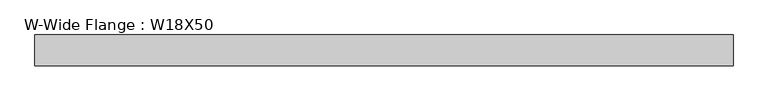
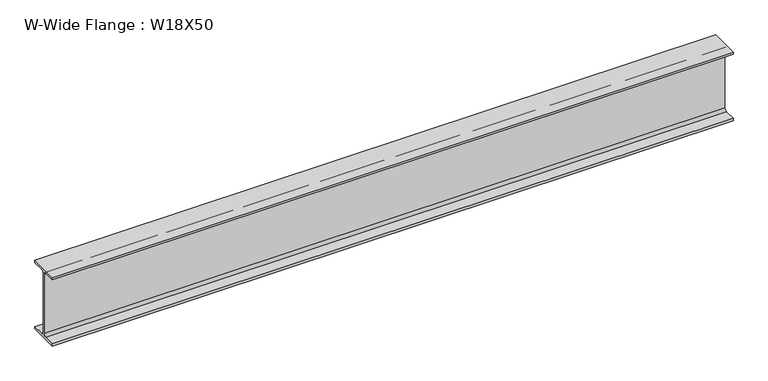
"""IFC4 building model written with IfcOpenShell, lengths in millimetres: beam geometry, W-Wide Flange : W18X50."""

from ifc_helpers import new_model, si_unit, point, frame, frame_2d, origin, place, context, project, spatial, polyline, circle_curve, trimmed, segment, composite_curve, outline, extrude, source, transform, mapped, element, save


def w_wide_flange_w18x50_e4b3ed06(model_context):
    return source(origin(), model_context, "Body", "SweptSolid", [
        extrude(outline(composite_curve([segment(polyline([(95.25, -214.122), (95.25, -228.6), (-95.25, -228.6), (-95.25, -214.122), (-21.7805, -214.122)]), True, "CONTINUOUS"), segment(trimmed(circle_curve(frame_2d((-21.7805, -196.85)), 17.272), [point((-21.7805, -214.122))], [point((-4.5085, -196.85))], True, "CARTESIAN"), True, "CONTINUOUS"), segment(polyline([(-4.5085, -196.85), (-4.5085, 196.85)]), True, "CONTINUOUS"), segment(trimmed(circle_curve(frame_2d((-21.7805, 196.85)), 17.272), [point((-4.5085, 196.85))], [point((-21.7805, 214.122))], True, "CARTESIAN"), True, "CONTINUOUS"), segment(polyline([(-21.7805, 214.122), (-95.25, 214.122), (-95.25, 228.6), (95.25, 228.6), (95.25, 214.122), (21.7805, 214.122)]), True, "CONTINUOUS"), segment(trimmed(circle_curve(frame_2d((21.7805, 196.85)), 17.272), [point((21.7805, 214.122))], [point((4.5085, 196.85))], True, "CARTESIAN"), True, "CONTINUOUS"), segment(polyline([(4.5085, 196.85), (4.5085, -196.85)]), True, "CONTINUOUS"), segment(trimmed(circle_curve(frame_2d((21.7805, -196.85)), 17.272), [point((4.5085, -196.85))], [point((21.7805, -214.122))], True, "CARTESIAN"), True, "CONTINUOUS"), segment(polyline([(21.7805, -214.122), (95.25, -214.122)]), True, "CONTINUOUS")], self_intersect=False)), frame((-2082.8, 0.0, 0.0), z_axis=(1.0, 0.0, 0.0), x_axis=(0.0, 1.0, 0.0)), (0.0, 0.0, 1.0), 4304.919),
    ])


if __name__ == "__main__":
    model = new_model("IFC4")
    model_context = context("Model", 3, world=origin())
    ifc_project = project(units=[si_unit("LENGTHUNIT", "METRE", prefix="MILLI")], contexts=[model_context])
    site = spatial("IfcSite", under=ifc_project)
    building = spatial("IfcBuilding", under=site)
    placement = place(None, origin())
    w_wide_flange_w18x50_shape = w_wide_flange_w18x50_e4b3ed06(model_context)
    element("IfcBeam", 1, ObjectType="W-Wide Flange : W18X50", at=placement, inside=building, context=model_context, shape_type="MappedRepresentation", body=[
        mapped(w_wide_flange_w18x50_shape, transform((0.0, 0.0, 0.0), x_axis=(1.0, 0.0, 0.0), y_axis=(0.0, 1.0, 0.0), z_axis=(0.0, 0.0, 1.0))),
    ])
    save(model, "model.ifc")

# Revit data of these elements
# Type "W-Wide Flange : W18X50"
#   Assembly Code = "B10"
#   W = 50
#   Length [instance default] = 5' - 0"
#   bf = 0' - 7 1/2"
#   d = 1' - 6"
#   k = 0' - 1 1/4"
#   k2 = 0' - 0.68"
#   tf = 0' - 0.57"
#   tw = 0' - 0.355"
#   A = 0.102083 SF
#   Structural Material [instance default] = Steel ASTM A992
# Element 1 (IfcBeam, "W-Wide Flange : W18X50")
#   Materials on its faces: "Steel ASTM A992"
# Materials
#   "Steel ASTM A992": class "Metal", colour RGB 199 199 199, transparency 0, Description = "Structural steel 50ksi", Cost = 0
